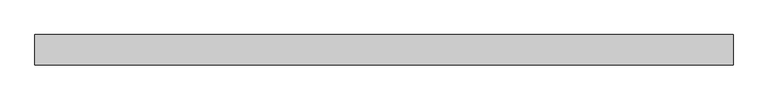
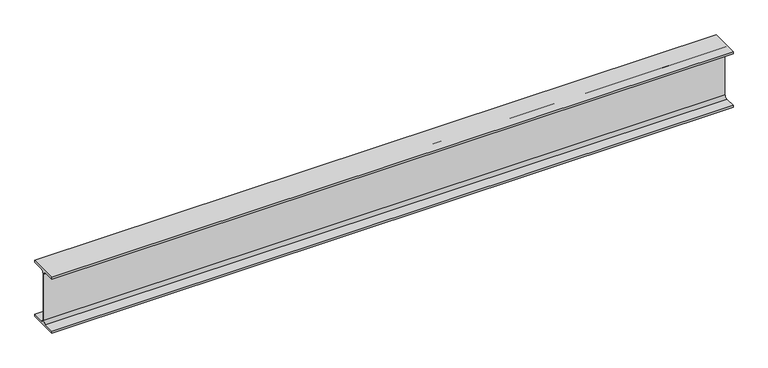
"""IFC4 building model written with IfcOpenShell, lengths in millimetres: beam geometry, 0912_Steel Framing_H-KSD3502 : H_SB_ASB_H-250x125x6x9."""

import ifcopenshell
import ifcopenshell.guid

model = None  # the IFC model being written
_history = None  # IfcOwnerHistory: only IFC2X3 demands one
_inside = {}  # id of a spatial element -> (the spatial element, [elements in it])
_under = {}  # id of a project, library or spatial element -> (it, [spatial elements below it])
_declared = {}  # id of a project -> (the project, [libraries it declares])
_typed = {}  # id of a type object -> (the type object, [elements of that type])
_made_of = {}  # id of a material, layer set ... -> (it, [elements and type objects made of it])


def new_model(schema):
    """Start an empty IFC model of exactly this schema.

    Asked for "IFC4X3", IfcOpenShell would pick the latest addendum, in which some entities
    have other attributes; the version numbers below select the first issue.
    IFC2X3 requires an IfcOwnerHistory on every rooted entity: one is made here for all.
    """
    global model, _history
    if schema == "IFC4X3":
        model = ifcopenshell.file(schema_version=(4, 3, 0, 0))
    else:
        model = ifcopenshell.file(schema=schema)
    _inside.clear()
    _under.clear()
    _declared.clear()
    _typed.clear()
    _made_of.clear()
    _history = None
    if model.schema == "IFC2X3":
        org = make("IfcOrganization", Name="unknown")
        user = make(
            "IfcPersonAndOrganization",
            ThePerson=make("IfcPerson", FamilyName="unknown"),
            TheOrganization=org,
        )
        app = make(
            "IfcApplication",
            ApplicationDeveloper=org,
            Version="unknown",
            ApplicationFullName="unknown",
            ApplicationIdentifier="unknown",
        )
        _history = make(
            "IfcOwnerHistory",
            OwningUser=user,
            OwningApplication=app,
            ChangeAction="ADDED",
            CreationDate=0,
        )
    return model


def make(cls, **values):
    """One entity of the class cls with the attributes given. An attribute that is None is left unset."""
    return model.create_entity(
        cls, **{name: value for name, value in values.items() if value is not None}
    )


def rooted(cls, **values):
    """An entity with a GlobalId (a new one), such as an element, a storey or a relation."""
    return make(cls, GlobalId=ifcopenshell.guid.new(), OwnerHistory=_history, **values)


def si_unit(unit_type, name, prefix=None):
    """IfcSIUnit, for example si_unit("LENGTHUNIT", "METRE", prefix="MILLI")."""
    return make("IfcSIUnit", UnitType=unit_type, Prefix=prefix, Name=name)


def assignment(units):
    """IfcUnitAssignment: the units of a project."""
    return None if units is None else make("IfcUnitAssignment", Units=units)


def point(xyz):
    """IfcCartesianPoint."""
    return None if xyz is None else make("IfcCartesianPoint", Coordinates=xyz)


def direction(xyz):
    """IfcDirection."""
    return None if xyz is None else make("IfcDirection", DirectionRatios=xyz)


def frame(location, z_axis=None, x_axis=None):
    """IfcAxis2Placement3D, a coordinate frame: its origin and axes. An axis left out is left unset."""
    return make(
        "IfcAxis2Placement3D",
        Location=point(location),
        Axis=direction(z_axis),
        RefDirection=direction(x_axis),
    )


def frame_2d(location, x_axis=None):
    """IfcAxis2Placement2D, a coordinate frame in the plane: its origin and x axis."""
    return make(
        "IfcAxis2Placement2D", Location=point(location), RefDirection=direction(x_axis)
    )


def origin():
    """The frame at (0, 0, 0) with its axes left unset."""
    return frame((0.0, 0.0, 0.0))


def place(relative_to, where):
    """IfcLocalPlacement: puts the frame where relative to a parent placement (None: the world)."""
    return make(
        "IfcLocalPlacement", PlacementRelTo=relative_to, RelativePlacement=where
    )


def context(
    kind, dimensions, precision=None, world=None, true_north=None, identifier=None
):
    """IfcGeometricRepresentationContext, for example the 3D "Model" context."""
    return make(
        "IfcGeometricRepresentationContext",
        ContextIdentifier=identifier,
        ContextType=kind,
        CoordinateSpaceDimension=dimensions,
        Precision=precision,
        WorldCoordinateSystem=world,
        TrueNorth=true_north,
    )


def project(units=None, contexts=None):
    """IfcProject with its units and contexts."""
    return rooted(
        "IfcProject",
        Name="project",
        RepresentationContexts=contexts,
        UnitsInContext=assignment(units),
    )


def spatial(cls, under=None, at=None, **own):
    """A site, building, storey or space (cls), placed at a placement, below another one or the project."""
    s = rooted(cls, ObjectPlacement=at, **own)
    if under is not None:
        _under.setdefault(under.id(), (under, []))[1].append(s)
    return s


def polyline(points):
    """IfcPolyline through the points."""
    return make("IfcPolyline", Points=[point(p) for p in points])


def circle_curve(where, radius):
    """IfcCircle in the frame where."""
    return make("IfcCircle", Position=where, Radius=radius)


def trimmed(basis, trim1, trim2, sense, master):
    """IfcTrimmedCurve: the piece of a basis curve between two trims."""
    return make(
        "IfcTrimmedCurve",
        BasisCurve=basis,
        Trim1=trim1,
        Trim2=trim2,
        SenseAgreement=sense,
        MasterRepresentation=master,
    )


def segment(curve, same_sense, transition):
    """IfcCompositeCurveSegment."""
    return make(
        "IfcCompositeCurveSegment",
        Transition=transition,
        SameSense=same_sense,
        ParentCurve=curve,
    )


def composite_curve(segments, self_intersect=None):
    """IfcCompositeCurve: segments joined end to end."""
    return make("IfcCompositeCurve", Segments=segments, SelfIntersect=self_intersect)


def outline(outer, holes=None, kind="AREA"):
    """IfcArbitraryClosedProfileDef: a profile drawn as a closed curve; with holes, ...WithVoids."""
    if holes is None:
        return make("IfcArbitraryClosedProfileDef", ProfileType=kind, OuterCurve=outer)
    return make(
        "IfcArbitraryProfileDefWithVoids",
        ProfileType=kind,
        OuterCurve=outer,
        InnerCurves=holes,
    )


def extrude(swept, where, along, depth):
    """IfcExtrudedAreaSolid: the profile swept, set in the frame where, extruded along a direction by depth."""
    return make(
        "IfcExtrudedAreaSolid",
        SweptArea=swept,
        Position=where,
        ExtrudedDirection=direction(along),
        Depth=depth,
    )


def shape(context_of_items, identifier, shape_type, items):
    """IfcShapeRepresentation: the items that make up one representation, for example the "Body"."""
    return make(
        "IfcShapeRepresentation",
        ContextOfItems=context_of_items,
        RepresentationIdentifier=identifier,
        RepresentationType=shape_type,
        Items=items,
    )


def source(mapping_origin, context_of_items, identifier, shape_type, items):
    """IfcRepresentationMap: a shape defined once, which mapped items show again and again."""
    return make(
        "IfcRepresentationMap",
        MappingOrigin=mapping_origin,
        MappedRepresentation=shape(context_of_items, identifier, shape_type, items),
    )


def transform(
    local_origin,
    x_axis=None,
    y_axis=None,
    z_axis=None,
    scale=None,
    scale2=None,
    scale3=None,
    uniform=True,
):
    """IfcCartesianTransformationOperator3D, or its non-uniform kind. x_axis, y_axis, z_axis: its Axis1, 2, 3."""
    if uniform:
        return make(
            "IfcCartesianTransformationOperator3D",
            Axis1=direction(x_axis),
            Axis2=direction(y_axis),
            LocalOrigin=point(local_origin),
            Scale=scale,
            Axis3=direction(z_axis),
        )
    return make(
        "IfcCartesianTransformationOperator3DnonUniform",
        Axis1=direction(x_axis),
        Axis2=direction(y_axis),
        LocalOrigin=point(local_origin),
        Scale=scale,
        Axis3=direction(z_axis),
        Scale2=scale2,
        Scale3=scale3,
    )


def mapped(mapping_source, mapping_target):
    """IfcMappedItem: shows the shape of a source again, moved by a transform."""
    return make(
        "IfcMappedItem", MappingSource=mapping_source, MappingTarget=mapping_target
    )


def made_of(thing, what):
    """Note that an element or type object is made of a material, layer set ...; save() writes the relation."""
    if what is not None:
        _made_of.setdefault(what.id(), (what, []))[1].append(thing)
    return thing


def element(
    cls,
    number,
    at=None,
    inside=None,
    cuts=None,
    type_object=None,
    material=None,
    context=None,
    identifier="Body",
    shape_type=None,
    held_by="IfcProductDefinitionShape",
    body=None,
    shapes=None,
    **own,
):
    """One element of the class cls, such as IfcWall. Its Tag is "e" and its number.

    at: its placement. inside: the storey or other place that contains it. cuts: it is an
    opening in that element (IfcRelVoidsElement). A single representation is given by context,
    identifier, shape_type and body (its items); several are given by shapes. held_by: the class
    of the entity that holds the representations. save() writes the other relations.
    """
    e = rooted(cls, Tag="e%d" % number, ObjectPlacement=at, **own)
    if body is not None:
        shapes = [shape(context, identifier, shape_type, body)]
    if shapes is not None:
        e.Representation = make(held_by, Representations=shapes)
    if inside is not None:
        _inside.setdefault(inside.id(), (inside, []))[1].append(e)
    if cuts is not None:
        rooted(
            "IfcRelVoidsElement", RelatingBuildingElement=cuts, RelatedOpeningElement=e
        )
    if type_object is not None:
        _typed.setdefault(type_object.id(), (type_object, []))[1].append(e)
    return made_of(e, material)


def aggregate(whole, parts):
    """IfcRelAggregates: a whole, such as a stair, and the parts it consists of."""
    return rooted("IfcRelAggregates", RelatingObject=whole, RelatedObjects=parts)


def save(model, path):
    """Write the relations noted so far, then the file.

    IfcRelAggregates (storeys below a building ...), IfcRelContainedInSpatialStructure (elements
    in a storey), IfcRelDefinesByType, IfcRelAssociatesMaterial and IfcRelDeclares: one each for
    every whole, place, type object, material and project.
    """
    for whole, parts in _under.values():
        aggregate(whole, parts)
    for where, things in _inside.values():
        rooted(
            "IfcRelContainedInSpatialStructure",
            RelatedElements=things,
            RelatingStructure=where,
        )
    for kind, things in _typed.values():
        rooted("IfcRelDefinesByType", RelatedObjects=things, RelatingType=kind)
    for what, things in _made_of.values():
        rooted("IfcRelAssociatesMaterial", RelatedObjects=things, RelatingMaterial=what)
    for by, libraries in _declared.values():
        rooted("IfcRelDeclares", RelatingContext=by, RelatedDefinitions=libraries)
    model.write(path)


def beam_eb669900(model_context):
    return source(origin(), model_context, "Body", "SweptSolid", [
        extrude(outline(composite_curve([segment(polyline([(62.5, -116.0), (62.5, -125.0), (-62.5, -125.0), (-62.5, -116.0), (-15.0, -116.0)]), True, "CONTINUOUS"), segment(trimmed(circle_curve(frame_2d((-15.0, -104.0)), 12.0), [point((-15.0, -116.0))], [point((-3.0, -104.0))], True, "CARTESIAN"), True, "CONTINUOUS"), segment(polyline([(-3.0, -104.0), (-3.0, 104.0)]), True, "CONTINUOUS"), segment(trimmed(circle_curve(frame_2d((-15.0, 104.0)), 12.0), [point((-3.0, 104.0))], [point((-15.0, 116.0))], True, "CARTESIAN"), True, "CONTINUOUS"), segment(polyline([(-15.0, 116.0), (-62.5, 116.0), (-62.5, 125.0), (62.5, 125.0), (62.5, 116.0), (15.0, 116.0)]), True, "CONTINUOUS"), segment(trimmed(circle_curve(frame_2d((15.0, 104.0)), 12.0), [point((15.0, 116.0))], [point((3.0, 104.0))], True, "CARTESIAN"), True, "CONTINUOUS"), segment(polyline([(3.0, 104.0), (3.0, -104.0)]), True, "CONTINUOUS"), segment(trimmed(circle_curve(frame_2d((15.0, -104.0)), 12.0), [point((3.0, -104.0))], [point((15.0, -116.0))], True, "CARTESIAN"), True, "CONTINUOUS"), segment(polyline([(15.0, -116.0), (62.5, -116.0)]), True, "CONTINUOUS")], self_intersect=False)), frame((-1404.8, 0.0, 0.0), z_axis=(1.0, 0.0, 0.0), x_axis=(0.0, 1.0, 0.0)), (0.0, 0.0, 1.0), 2892.0999994),
    ])


if __name__ == "__main__":
    model = new_model("IFC4")
    model_context = context("Model", 3, world=origin())
    ifc_project = project(units=[si_unit("LENGTHUNIT", "METRE", prefix="MILLI")], contexts=[model_context])
    site = spatial("IfcSite", under=ifc_project)
    building = spatial("IfcBuilding", under=site)
    placement = place(None, origin())
    beam_shape = beam_eb669900(model_context)
    element("IfcBeam", 1, ObjectType="0912_Steel Framing_H-KSD3502 : H_SB_ASB_H-250x125x6x9", at=placement, inside=building, context=model_context, shape_type="MappedRepresentation", body=[
        mapped(beam_shape, transform((0.0, 0.0, 0.0), x_axis=(1.0, 0.0, 0.0), y_axis=(0.0, 1.0, 0.0), z_axis=(0.0, 0.0, 1.0))),
    ])
    save(model, "model.ifc")

# Revit data of these elements
# Type "0912_Steel Framing_H-KSD3502 : H_SB_ASB_H-250x125x6x9"
#   H_WM Code_1 = "S01AA003-00001 | Main Steel Structure Fabrication Work | Shelter/Building | Light Steel - Standard (30KG/M>Weight) | Material: (   )"
#   H_WM Code_2 = "S03AA029-00001 | Main Steel Structure Erection Work | Shelter/Building | Light Steel (30KG/M>Weight) | Material: (   )"
#   H_WM Code_3 = "S01AA010-00001 | Main Steel Structure Fabrication Work | Shelter/Building | Steel Painting/Coating | for Non-Fireproofed Steel Surface, Surface Preparation, Primer, Second & Final Coat | Material: (   )"
#   H_Q'ty Cal Type Tag = "SB-Q2"
#   Width = 12.5 cm
#   Web Thickness = 0.6 cm
#   Web Fillet = 1.2 cm
#   Warping Constant = 42539.8 cm⁶
#   W = 0
#   Torsional Moment of Inertia = 7.8102 cm⁴
#   Section Area = 37.66 cm²
#   Plastic Modulus weak axis = 73.1 cm³
#   Plastic Modulus strong axis = 366.0 cm³
#   Perimeter = 0.97 m²/m
#   Nominal Weight = 29.60 kgf/m
#   Moment of Inertia weak axis = 294.00 cm⁴
#   Moment of Inertia strong axis = 4050.00 cm⁴
#   Height = 25.0 cm
#   Flange Thickness = 0.9 cm
#   Elastic Modulus weak axis = 47.0 cm³
#   Elastic Modulus strong axis = 324.0 cm³
#   Centroid Vertical = 12.5 cm
#   Centroid Horizontal = 6.25 cm
#   Ix = 40500000
#   Length [instance default] = 1.5240 m
#   Zx = 366000
#   b = 0.1250 m
#   h = 0.2500 m
#   r = 0.0120 m
#   s = 0.0060 m
#   t = 0.0090 m
#   A = 0.003766 m²
#   Structural Material [instance default] = Steel, 45-345
#   Assembly Code = ""
# Element 1 (IfcBeam, "0912_Steel Framing_H-KSD3502 : H_SB_ASB_H-250x125x6x9")
#   Structural Material = none
# Materials
#   "Steel, 45-345": class "Metal", colour RGB 189 187 185, transparency 0, Description = "Steel 345 MPa", Cost = 0
